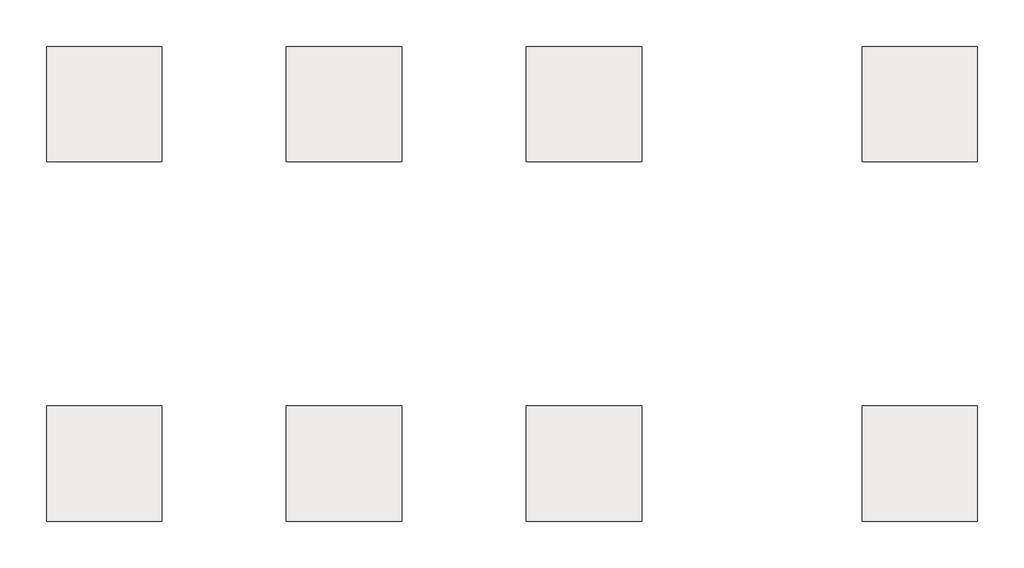
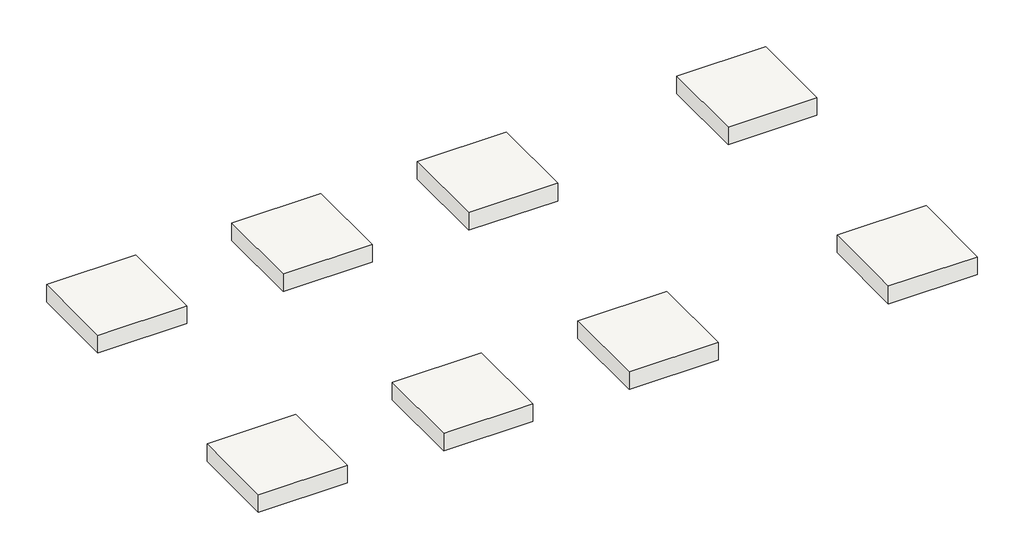
# Not in any storey: 8 slabs.
"""IFC4 building model written with IfcOpenShell, lengths in millimetres."""

import ifcopenshell
import ifcopenshell.guid

model = None  # the IFC model being written
_history = None  # IfcOwnerHistory: only IFC2X3 demands one
_inside = {}  # id of a spatial element -> (the spatial element, [elements in it])
_under = {}  # id of a project, library or spatial element -> (it, [spatial elements below it])
_declared = {}  # id of a project -> (the project, [libraries it declares])
_typed = {}  # id of a type object -> (the type object, [elements of that type])
_made_of = {}  # id of a material, layer set ... -> (it, [elements and type objects made of it])


def new_model(schema):
    """Start an empty IFC model of exactly this schema.

    Asked for "IFC4X3", IfcOpenShell would pick the latest addendum, in which some entities
    have other attributes; the version numbers below select the first issue.
    IFC2X3 requires an IfcOwnerHistory on every rooted entity: one is made here for all.
    """
    global model, _history
    if schema == "IFC4X3":
        model = ifcopenshell.file(schema_version=(4, 3, 0, 0))
    else:
        model = ifcopenshell.file(schema=schema)
    _inside.clear()
    _under.clear()
    _declared.clear()
    _typed.clear()
    _made_of.clear()
    _history = None
    if model.schema == "IFC2X3":
        org = make("IfcOrganization", Name="unknown")
        user = make(
            "IfcPersonAndOrganization",
            ThePerson=make("IfcPerson", FamilyName="unknown"),
            TheOrganization=org,
        )
        app = make(
            "IfcApplication",
            ApplicationDeveloper=org,
            Version="unknown",
            ApplicationFullName="unknown",
            ApplicationIdentifier="unknown",
        )
        _history = make(
            "IfcOwnerHistory",
            OwningUser=user,
            OwningApplication=app,
            ChangeAction="ADDED",
            CreationDate=0,
        )
    return model


def make(cls, **values):
    """One entity of the class cls with the attributes given. An attribute that is None is left unset."""
    return model.create_entity(
        cls, **{name: value for name, value in values.items() if value is not None}
    )


def rooted(cls, **values):
    """An entity with a GlobalId (a new one), such as an element, a storey or a relation."""
    return make(cls, GlobalId=ifcopenshell.guid.new(), OwnerHistory=_history, **values)


def si_unit(unit_type, name, prefix=None):
    """IfcSIUnit, for example si_unit("LENGTHUNIT", "METRE", prefix="MILLI")."""
    return make("IfcSIUnit", UnitType=unit_type, Prefix=prefix, Name=name)


def assignment(units):
    """IfcUnitAssignment: the units of a project."""
    return None if units is None else make("IfcUnitAssignment", Units=units)


def point(xyz):
    """IfcCartesianPoint."""
    return None if xyz is None else make("IfcCartesianPoint", Coordinates=xyz)


def direction(xyz):
    """IfcDirection."""
    return None if xyz is None else make("IfcDirection", DirectionRatios=xyz)


def frame(location, z_axis=None, x_axis=None):
    """IfcAxis2Placement3D, a coordinate frame: its origin and axes. An axis left out is left unset."""
    return make(
        "IfcAxis2Placement3D",
        Location=point(location),
        Axis=direction(z_axis),
        RefDirection=direction(x_axis),
    )


def origin():
    """The frame at (0, 0, 0) with its axes left unset."""
    return frame((0.0, 0.0, 0.0))


def place(relative_to, where):
    """IfcLocalPlacement: puts the frame where relative to a parent placement (None: the world)."""
    return make(
        "IfcLocalPlacement", PlacementRelTo=relative_to, RelativePlacement=where
    )


def context(
    kind, dimensions, precision=None, world=None, true_north=None, identifier=None
):
    """IfcGeometricRepresentationContext, for example the 3D "Model" context."""
    return make(
        "IfcGeometricRepresentationContext",
        ContextIdentifier=identifier,
        ContextType=kind,
        CoordinateSpaceDimension=dimensions,
        Precision=precision,
        WorldCoordinateSystem=world,
        TrueNorth=true_north,
    )


def project(units=None, contexts=None):
    """IfcProject with its units and contexts."""
    return rooted(
        "IfcProject",
        Name="project",
        RepresentationContexts=contexts,
        UnitsInContext=assignment(units),
    )


def spatial(cls, under=None, at=None, **own):
    """A site, building, storey or space (cls), placed at a placement, below another one or the project."""
    s = rooted(cls, ObjectPlacement=at, **own)
    if under is not None:
        _under.setdefault(under.id(), (under, []))[1].append(s)
    return s


def polyline(points):
    """IfcPolyline through the points."""
    return make("IfcPolyline", Points=[point(p) for p in points])


def outline(outer, holes=None, kind="AREA"):
    """IfcArbitraryClosedProfileDef: a profile drawn as a closed curve; with holes, ...WithVoids."""
    if holes is None:
        return make("IfcArbitraryClosedProfileDef", ProfileType=kind, OuterCurve=outer)
    return make(
        "IfcArbitraryProfileDefWithVoids",
        ProfileType=kind,
        OuterCurve=outer,
        InnerCurves=holes,
    )


def extrude(swept, where, along, depth):
    """IfcExtrudedAreaSolid: the profile swept, set in the frame where, extruded along a direction by depth."""
    return make(
        "IfcExtrudedAreaSolid",
        SweptArea=swept,
        Position=where,
        ExtrudedDirection=direction(along),
        Depth=depth,
    )


def faces_of(points, faces, orient=None, outer=None):
    """IfcFace entities. A face is a list of loops; a loop is a list of indices into points, from 0.

    orient and outer hold one flag for each loop. By default every Orientation is true, the
    first loop of a face is its IfcFaceOuterBound and the others are IfcFaceBound.
    """
    made = []
    for i, loops in enumerate(faces):
        bounds = []
        for j, loop in enumerate(loops):
            is_outer = j == 0 if outer is None else outer[i][j]
            bounds.append(
                make(
                    "IfcFaceOuterBound" if is_outer else "IfcFaceBound",
                    Bound=make("IfcPolyLoop", Polygon=[points[k] for k in loop]),
                    Orientation=True if orient is None else orient[i][j],
                )
            )
        made.append(make("IfcFace", Bounds=bounds))
    return made


def faceted_brep(points, faces, orient=None, outer=None, voids=None):
    """IfcFacetedBrep: a solid bounded by flat faces; with voids (closed shells), ...WithVoids."""
    shared = [point(p) for p in points]
    hull = make("IfcClosedShell", CfsFaces=faces_of(shared, faces, orient, outer))
    if voids is None:
        return make("IfcFacetedBrep", Outer=hull)
    return make(
        "IfcFacetedBrepWithVoids",
        Outer=hull,
        Voids=[
            make(cls, CfsFaces=faces_of(shared, fs, o, b)) for cls, fs, o, b in voids
        ],
    )


def shape(context_of_items, identifier, shape_type, items):
    """IfcShapeRepresentation: the items that make up one representation, for example the "Body"."""
    return make(
        "IfcShapeRepresentation",
        ContextOfItems=context_of_items,
        RepresentationIdentifier=identifier,
        RepresentationType=shape_type,
        Items=items,
    )


def source(mapping_origin, context_of_items, identifier, shape_type, items):
    """IfcRepresentationMap: a shape defined once, which mapped items show again and again."""
    return make(
        "IfcRepresentationMap",
        MappingOrigin=mapping_origin,
        MappedRepresentation=shape(context_of_items, identifier, shape_type, items),
    )


def transform(
    local_origin,
    x_axis=None,
    y_axis=None,
    z_axis=None,
    scale=None,
    scale2=None,
    scale3=None,
    uniform=True,
):
    """IfcCartesianTransformationOperator3D, or its non-uniform kind. x_axis, y_axis, z_axis: its Axis1, 2, 3."""
    if uniform:
        return make(
            "IfcCartesianTransformationOperator3D",
            Axis1=direction(x_axis),
            Axis2=direction(y_axis),
            LocalOrigin=point(local_origin),
            Scale=scale,
            Axis3=direction(z_axis),
        )
    return make(
        "IfcCartesianTransformationOperator3DnonUniform",
        Axis1=direction(x_axis),
        Axis2=direction(y_axis),
        LocalOrigin=point(local_origin),
        Scale=scale,
        Axis3=direction(z_axis),
        Scale2=scale2,
        Scale3=scale3,
    )


def mapped(mapping_source, mapping_target):
    """IfcMappedItem: shows the shape of a source again, moved by a transform."""
    return make(
        "IfcMappedItem", MappingSource=mapping_source, MappingTarget=mapping_target
    )


def made_of(thing, what):
    """Note that an element or type object is made of a material, layer set ...; save() writes the relation."""
    if what is not None:
        _made_of.setdefault(what.id(), (what, []))[1].append(thing)
    return thing


def element(
    cls,
    number,
    at=None,
    inside=None,
    cuts=None,
    type_object=None,
    material=None,
    context=None,
    identifier="Body",
    shape_type=None,
    held_by="IfcProductDefinitionShape",
    body=None,
    shapes=None,
    **own,
):
    """One element of the class cls, such as IfcWall. Its Tag is "e" and its number.

    at: its placement. inside: the storey or other place that contains it. cuts: it is an
    opening in that element (IfcRelVoidsElement). A single representation is given by context,
    identifier, shape_type and body (its items); several are given by shapes. held_by: the class
    of the entity that holds the representations. save() writes the other relations.
    """
    e = rooted(cls, Tag="e%d" % number, ObjectPlacement=at, **own)
    if body is not None:
        shapes = [shape(context, identifier, shape_type, body)]
    if shapes is not None:
        e.Representation = make(held_by, Representations=shapes)
    if inside is not None:
        _inside.setdefault(inside.id(), (inside, []))[1].append(e)
    if cuts is not None:
        rooted(
            "IfcRelVoidsElement", RelatingBuildingElement=cuts, RelatedOpeningElement=e
        )
    if type_object is not None:
        _typed.setdefault(type_object.id(), (type_object, []))[1].append(e)
    return made_of(e, material)


def aggregate(whole, parts):
    """IfcRelAggregates: a whole, such as a stair, and the parts it consists of."""
    return rooted("IfcRelAggregates", RelatingObject=whole, RelatedObjects=parts)


def save(model, path):
    """Write the relations noted so far, then the file.

    IfcRelAggregates (storeys below a building ...), IfcRelContainedInSpatialStructure (elements
    in a storey), IfcRelDefinesByType, IfcRelAssociatesMaterial and IfcRelDeclares: one each for
    every whole, place, type object, material and project.
    """
    for whole, parts in _under.values():
        aggregate(whole, parts)
    for where, things in _inside.values():
        rooted(
            "IfcRelContainedInSpatialStructure",
            RelatedElements=things,
            RelatingStructure=where,
        )
    for kind, things in _typed.values():
        rooted("IfcRelDefinesByType", RelatedObjects=things, RelatingType=kind)
    for what, things in _made_of.values():
        rooted("IfcRelAssociatesMaterial", RelatedObjects=things, RelatingMaterial=what)
    for by, libraries in _declared.values():
        rooted("IfcRelDeclares", RelatingContext=by, RelatedDefinitions=libraries)
    model.write(path)


def ft211_footing_rectangular_r0_ft211_footing_rectangular_5fe39465(model_context):
    return source(origin(), model_context, "Body", "SweptSolid", [
        extrude(outline(polyline([(1200.0, 1200.0), (1200.0, -1200.0), (-1200.0, -1200.0), (-1200.0, 1200.0), (1200.0, 1200.0)])), frame((0.0, 0.0, -500.0), z_axis=(0.0, 0.0, 1.0), x_axis=(1.0, 0.0, 0.0)), (0.0, 0.0, 1.0), 500.0),
    ])


model = new_model("IFC4")

# Units and contexts
model_context = context("Model", 3, world=origin())
ifc_project = project(units=[si_unit("LENGTHUNIT", "METRE", prefix="MILLI")], contexts=[model_context])

# Site, building
site = spatial("IfcSite", under=ifc_project)
building = spatial("IfcBuilding", under=site)

# Slabs
placement = place(None, origin())
element("IfcSlab", 1, ObjectType="FT211-Footing-Rectangular_R0 : FT211_Footing-Rectangular_2400x2400x500_F1", at=placement, inside=building, context=model_context, shape_type="SweptSolid", body=[
    extrude(outline(polyline([(11200.0, 22199.5208589), (11200.0, 19799.5208589), (8800.0, 19799.5208589), (8800.0, 22199.5208589), (11200.0, 22199.5208589)])), frame((0.0, 0.0, -1800.0), z_axis=(0.0, 0.0, 1.0), x_axis=(1.0, 0.0, 0.0)), (0.0, 0.0, 1.0), 500.0),
])
element("IfcSlab", 2, ObjectType="FT211-Footing-Rectangular_R0 : FT211_Footing-Rectangular_2400x2400x500_F1", at=placement, inside=building, context=model_context, shape_type="SweptSolid", body=[
    extrude(outline(polyline([(6200.0, 22199.5208589), (6200.0, 19799.5208589), (3800.0, 19799.5208589), (3800.0, 22199.5208589), (6200.0, 22199.5208589)])), frame((0.0, 0.0, -1800.0), z_axis=(0.0, 0.0, 1.0), x_axis=(1.0, 0.0, 0.0)), (0.0, 0.0, 1.0), 500.0),
])
element("IfcSlab", 3, ObjectType="FT211-Footing-Rectangular_R0 : FT211_Footing-Rectangular_2400x2400x500_F1", at=placement, inside=building, context=model_context, shape_type="Brep", body=[
    faceted_brep([(1200.0, 22199.5208589, -1300.0), (-1200.0, 22199.5208589, -1300.0), (-1200.0, 19799.5208589, -1300.0), (1200.0, 19799.5208589, -1300.0), (1200.0, 22199.5208589, -1800.0), (1200.0, 21958.6768195, -1800.0), (1200.0, 19799.5208589, -1800.0), (-959.1559606, 19799.5208589, -1800.0), (-1200.0, 19799.5208589, -1800.0), (-1200.0, 22199.5208589, -1800.0)], [[[0, 1, 2, 3]], [[4, 5, 6, 7, 8, 9]], [[1, 0, 4, 9]], [[2, 1, 9, 8]], [[3, 2, 8, 7, 6]], [[0, 3, 6, 5, 4]]]),
])
element("IfcSlab", 4, ObjectType="FT211-Footing-Rectangular_R0 : FT211_Footing-Rectangular_2400x2400x500_F1", at=placement, inside=building, context=model_context, shape_type="SweptSolid", body=[
    extrude(outline(polyline([(1200.0, 14699.5208589), (1200.0, 12299.5208589), (-1200.0, 12299.5208589), (-1200.0, 14699.5208589), (1200.0, 14699.5208589)])), frame((0.0, 0.0, -1800.0), z_axis=(0.0, 0.0, 1.0), x_axis=(1.0, 0.0, 0.0)), (0.0, 0.0, 1.0), 500.0),
])
element("IfcSlab", 5, ObjectType="FT211-Footing-Rectangular_R0 : FT211_Footing-Rectangular_2400x2400x500_F1", at=placement, inside=building, context=model_context, shape_type="SweptSolid", body=[
    extrude(outline(polyline([(18200.0, 22199.5208589), (18200.0, 19799.5208589), (15800.0, 19799.5208589), (15800.0, 22199.5208589), (18200.0, 22199.5208589)])), frame((0.0, 0.0, -1800.0), z_axis=(0.0, 0.0, 1.0), x_axis=(1.0, 0.0, 0.0)), (0.0, 0.0, 1.0), 500.0),
])
ft211_footing_rectangular_r0_ft211_footing_rectangular_shape = ft211_footing_rectangular_r0_ft211_footing_rectangular_5fe39465(model_context)
element("IfcSlab", 6, ObjectType="FT211-Footing-Rectangular_R0 : FT211_Footing-Rectangular_2400x2400x500_F1", at=placement, inside=building, context=model_context, shape_type="MappedRepresentation", body=[
    mapped(ft211_footing_rectangular_r0_ft211_footing_rectangular_shape, transform((5000.0, 13499.5208589, -1300.0), x_axis=(1.0, 0.0, 0.0), y_axis=(0.0, 1.0, 0.0), z_axis=(0.0, 0.0, 1.0))),
])
element("IfcSlab", 7, ObjectType="FT211-Footing-Rectangular_R0 : FT211_Footing-Rectangular_2400x2400x500_F1", at=placement, inside=building, context=model_context, shape_type="MappedRepresentation", body=[
    mapped(ft211_footing_rectangular_r0_ft211_footing_rectangular_shape, transform((10000.0, 13499.5208589, -1300.0), x_axis=(1.0, 0.0, 0.0), y_axis=(0.0, 1.0, 0.0), z_axis=(0.0, 0.0, 1.0))),
])
element("IfcSlab", 8, ObjectType="FT211-Footing-Rectangular_R0 : FT211_Footing-Rectangular_2400x2400x500_F1", at=placement, inside=building, context=model_context, shape_type="MappedRepresentation", body=[
    mapped(ft211_footing_rectangular_r0_ft211_footing_rectangular_shape, transform((17000.0, 13499.5208589, -1300.0), x_axis=(1.0, 0.0, 0.0), y_axis=(0.0, 1.0, 0.0), z_axis=(0.0, 0.0, 1.0))),
])

save(model, "model.ifc")

# Revit data of these elements
# Project information
#   Building Name = "MAIN GATE SECURITY BUILDING"
#   Project Status = "Project Status"
#   Client Name = "현대엔지니어링"
#   Project Address = "서울시 종로구 율곡로 75(계동)"
#   Project Name = "Therma Visayas Energy Project"
#   Project Number = "-"
# Grids (mm)
#   "A": line (0, 24502.793) -> (0, 11308.625)
#   "B": line (5000, 24502.793) -> (5000, 11308.625)
#   "C": line (10000, 24502.793) -> (10000, 11308.625)
#   "1": line (-3860.098, 13499.521) -> (12441.468, 13499.521)
#   "2": line (-3860.098, 20999.521) -> (12441.468, 20999.521)
# Type "FT211-Footing-Rectangular_R0 : FT211_Footing-Rectangular_2400x2400x500_F1"
#   Top bar = "D25@300"
#   Description = "UG Shallow Foundation"
#   Bottom bar = "D20@300"
#   Width = 2400 mm
#   Length = 2400 mm
#   Foundation Thickness = 500 mm
#   Structural Material [instance default] = A03AC032-00007_Structural Concrete_Type1_25MPa-30Mpa
#   Assembly Code = ""
# Elements 1, 2, 3, 4, 6, 7 (IfcSlab, "FT211-Footing-Rectangular_R0 : FT211_Footing-Rectangular_2400x2400x500_F1")
#   Comments = ""
#   Mark = "F1"
#   F01) Building Name = "Main Gate House"
#   F11) Project Building Tag_Type-1 = "Common"
#   F12) Project Building Tag_Type-2 = "Common"
#   F13) Project Facility Code = "Facility Code"
#   F21) Structural Type = "Concrete"
#   F31) Standard Building Code = "IBC"
#   F41) Discipline = "AR"
#   F51) Plan Start Date-Engineering = "2015-01-01"
#   F52) Plan Finish Date-Engineering = "2015-12-31"
#   F53) Duration = "365"
#   F54) Actual Start Date-Engineering = "2015-01-01"
#   F55) Actual Finish Date-Engineering = "2015-12-31"
#   F61) Plan Start Date-Construction = "2016-08-19"
#   F62) Plan Finish Date-Construction = "2017-01-31"
#   F64) Actual Start Date-Construction = "2016-08-19"
#   F63) Duration = "202"
#   F65) Actual Finish Date-Construction = "2017-01-31"
#   F91) Plant Type = "CFPP"
#   F92) KKS Structures, Building = "UYF"
#   P01) Project Name = "TVEP"
#   P02) Project Configuration = "CFB Boiler x 2(Foster Wheeler) + STG x 2(Alstom, 150MW)"
#   P03) Project Abbreviation = "TVEP"
#   P04) Project Code = "BEPH1402"
#   P05) Project Stage = "In operation"
#   P06) Project Location = "Sito Looc, Barangay Bato, Toledo City in Philippines"
#   P07) Project Owner = "Therma Visayas, Inc."
#   P08) Project O.E = "Flour"
#   P09) Project Schedule = "ITB Issueing Date : 2013.07.30\r\nSite Survey : 2013.08.19-20\r\nBid Closing Date : 2013.11.29\r\nPreferred Bidder Notice 접수 : 2014.04.27\r\nTarget award date : 2014 05\r\nLOA 접수 : 2014.05.21\r\nSigning Ceremony : 2014.05.30"
#   P10) Basic Wind Speed = "55.6 m/s"
#   P11) Seismic = "NSCP 2010, Zone 4 (PGA : 0.4g)"
#   P12) Soil = "Sc"
#   P13) Soil Capacity = "100kN/m2"
#   P14) Pile Capacity = "PHC(D400) : 1200kN"
#   W00) Work Master Code = "A03AC032-00007"
#   W01) Work Master_Lv1 = "Concrete Work"
#   W02) Work Master_Lv2 = "Substructure Work"
#   W03) Work Master_Spec.1 = "Cement Type-1"
#   W04) Work Master_Spec.2 = "25MPa < F'c (Cylinder Strength) ≤ 30MPa"
#   W11) Activity ID = "C02AGB010"
#   W12) Activity Name = "Main Gate Security Building - Building Foundation"
#   W13) Plan Start Date = "2016-08-19"
#   W14) Plan Finish Date = "2016-09-22"
#   W15) Duration = "26"
#   W16) Actual Start Date = "2016-08-19"
#   W17) Actual Finish Date = "2016-09-22"
#   R02) Unit Price = 0
#   Structural Material = A03AC032-00007_Structural Concrete_Type1_25MPa-30Mpa
#   Phase Created = New Construction
#   Materials on its faces: "A03AC032-00007_Structural Concrete_Type1_25MPa-30Mpa"
# Elements 5, 8 (IfcSlab, "FT211-Footing-Rectangular_R0 : FT211_Footing-Rectangular_2400x2400x500_F1")
#   Comments = ""
#   F01) Building Name = "Main Gate House"
#   F11) Project Building Tag_Type-1 = "Common"
#   F12) Project Building Tag_Type-2 = "Common"
#   F13) Project Facility Code = "Facility Code"
#   F21) Structural Type = "Concrete"
#   F31) Standard Building Code = "IBC"
#   F41) Discipline = "AR"
#   F51) Plan Start Date-Engineering = "2015-01-01"
#   F52) Plan Finish Date-Engineering = "2015-12-31"
#   F53) Duration = "365"
#   F54) Actual Start Date-Engineering = "2015-01-01"
#   F55) Actual Finish Date-Engineering = "2015-12-31"
#   F61) Plan Start Date-Construction = "2016-08-19"
#   F62) Plan Finish Date-Construction = "2017-01-31"
#   F64) Actual Start Date-Construction = "2016-08-19"
#   F63) Duration = "202"
#   F65) Actual Finish Date-Construction = "2017-01-31"
#   F91) Plant Type = "CFPP"
#   F92) KKS Structures, Building = "UYF"
#   P01) Project Name = "TVEP"
#   P02) Project Configuration = "CFB Boiler x 2(Foster Wheeler) + STG x 2(Alstom, 150MW)"
#   P03) Project Abbreviation = "TVEP"
#   P04) Project Code = "BEPH1402"
#   P05) Project Stage = "In operation"
#   P06) Project Location = "Sito Looc, Barangay Bato, Toledo City in Philippines"
#   P07) Project Owner = "Therma Visayas, Inc."
#   P08) Project O.E = "Flour"
#   P09) Project Schedule = "ITB Issueing Date : 2013.07.30\r\nSite Survey : 2013.08.19-20\r\nBid Closing Date : 2013.11.29\r\nPreferred Bidder Notice 접수 : 2014.04.27\r\nTarget award date : 2014 05\r\nLOA 접수 : 2014.05.21\r\nSigning Ceremony : 2014.05.30"
#   P10) Basic Wind Speed = "55.6 m/s"
#   P11) Seismic = "NSCP 2010, Zone 4 (PGA : 0.4g)"
#   P12) Soil = "Sc"
#   P13) Soil Capacity = "100kN/m2"
#   P14) Pile Capacity = "PHC(D400) : 1200kN"
#   W00) Work Master Code = "A03AC032-00007"
#   W01) Work Master_Lv1 = "Concrete Work"
#   W02) Work Master_Lv2 = "Substructure Work"
#   W03) Work Master_Spec.1 = "Cement Type-1"
#   W04) Work Master_Spec.2 = "25MPa < F'c (Cylinder Strength) ≤ 30MPa"
#   W11) Activity ID = "C02AGB010"
#   W12) Activity Name = "Main Gate Security Building - Building Foundation"
#   W13) Plan Start Date = "2016-08-19"
#   W14) Plan Finish Date = "2016-09-22"
#   W15) Duration = "26"
#   W16) Actual Start Date = "2016-08-19"
#   W17) Actual Finish Date = "2016-09-22"
#   R02) Unit Price = 0
#   Structural Material = A03AC032-00007_Structural Concrete_Type1_25MPa-30Mpa
#   Phase Created = New Construction
#   Materials on its faces: "A03AC032-00007_Structural Concrete_Type1_25MPa-30Mpa"
# Materials
#   "A03AC032-00007_Structural Concrete_Type1_25MPa-30Mpa": class "Concrete", colour RGB 176 176 176, transparency 0, Keynote = "09910.A1", Description = "Reinf. Conc.", W00) Work Master Code = "A03AC032-00007", W01) Work Master_Lv1 = "Concrete Work", W02) Work Master_Lv2 = "Substructure Work", W03) Work Master_Spec.1 = "Structural Concrete", W04) Work Master_Spec.2 = "Cement Type-1", W05) Work Master_Spec.3 = "25MPa < F'c (Cylinder Strength) ≤ 30MPa", Cost = 0
